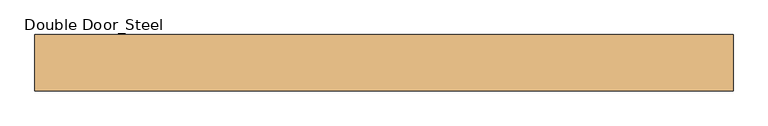
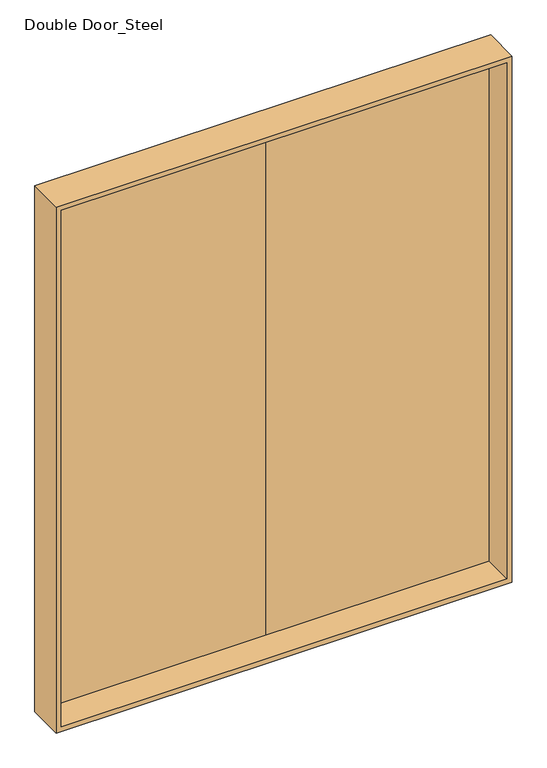
"""IFC4 building model written with IfcOpenShell, lengths in millimetres: door geometry, Double Door_Steel : H_DR_AR_B12_Double Door_Steel_W3100xH3780_FSD4."""

import ifcopenshell
import ifcopenshell.guid

model = None  # the IFC model being written
_history = None  # IfcOwnerHistory: only IFC2X3 demands one
_inside = {}  # id of a spatial element -> (the spatial element, [elements in it])
_under = {}  # id of a project, library or spatial element -> (it, [spatial elements below it])
_declared = {}  # id of a project -> (the project, [libraries it declares])
_typed = {}  # id of a type object -> (the type object, [elements of that type])
_made_of = {}  # id of a material, layer set ... -> (it, [elements and type objects made of it])


def new_model(schema):
    """Start an empty IFC model of exactly this schema.

    Asked for "IFC4X3", IfcOpenShell would pick the latest addendum, in which some entities
    have other attributes; the version numbers below select the first issue.
    IFC2X3 requires an IfcOwnerHistory on every rooted entity: one is made here for all.
    """
    global model, _history
    if schema == "IFC4X3":
        model = ifcopenshell.file(schema_version=(4, 3, 0, 0))
    else:
        model = ifcopenshell.file(schema=schema)
    _inside.clear()
    _under.clear()
    _declared.clear()
    _typed.clear()
    _made_of.clear()
    _history = None
    if model.schema == "IFC2X3":
        org = make("IfcOrganization", Name="unknown")
        user = make(
            "IfcPersonAndOrganization",
            ThePerson=make("IfcPerson", FamilyName="unknown"),
            TheOrganization=org,
        )
        app = make(
            "IfcApplication",
            ApplicationDeveloper=org,
            Version="unknown",
            ApplicationFullName="unknown",
            ApplicationIdentifier="unknown",
        )
        _history = make(
            "IfcOwnerHistory",
            OwningUser=user,
            OwningApplication=app,
            ChangeAction="ADDED",
            CreationDate=0,
        )
    return model


def make(cls, **values):
    """One entity of the class cls with the attributes given. An attribute that is None is left unset."""
    return model.create_entity(
        cls, **{name: value for name, value in values.items() if value is not None}
    )


def rooted(cls, **values):
    """An entity with a GlobalId (a new one), such as an element, a storey or a relation."""
    return make(cls, GlobalId=ifcopenshell.guid.new(), OwnerHistory=_history, **values)


def si_unit(unit_type, name, prefix=None):
    """IfcSIUnit, for example si_unit("LENGTHUNIT", "METRE", prefix="MILLI")."""
    return make("IfcSIUnit", UnitType=unit_type, Prefix=prefix, Name=name)


def assignment(units):
    """IfcUnitAssignment: the units of a project."""
    return None if units is None else make("IfcUnitAssignment", Units=units)


def point(xyz):
    """IfcCartesianPoint."""
    return None if xyz is None else make("IfcCartesianPoint", Coordinates=xyz)


def direction(xyz):
    """IfcDirection."""
    return None if xyz is None else make("IfcDirection", DirectionRatios=xyz)


def frame(location, z_axis=None, x_axis=None):
    """IfcAxis2Placement3D, a coordinate frame: its origin and axes. An axis left out is left unset."""
    return make(
        "IfcAxis2Placement3D",
        Location=point(location),
        Axis=direction(z_axis),
        RefDirection=direction(x_axis),
    )


def origin():
    """The frame at (0, 0, 0) with its axes left unset."""
    return frame((0.0, 0.0, 0.0))


def place(relative_to, where):
    """IfcLocalPlacement: puts the frame where relative to a parent placement (None: the world)."""
    return make(
        "IfcLocalPlacement", PlacementRelTo=relative_to, RelativePlacement=where
    )


def context(
    kind, dimensions, precision=None, world=None, true_north=None, identifier=None
):
    """IfcGeometricRepresentationContext, for example the 3D "Model" context."""
    return make(
        "IfcGeometricRepresentationContext",
        ContextIdentifier=identifier,
        ContextType=kind,
        CoordinateSpaceDimension=dimensions,
        Precision=precision,
        WorldCoordinateSystem=world,
        TrueNorth=true_north,
    )


def project(units=None, contexts=None):
    """IfcProject with its units and contexts."""
    return rooted(
        "IfcProject",
        Name="project",
        RepresentationContexts=contexts,
        UnitsInContext=assignment(units),
    )


def spatial(cls, under=None, at=None, **own):
    """A site, building, storey or space (cls), placed at a placement, below another one or the project."""
    s = rooted(cls, ObjectPlacement=at, **own)
    if under is not None:
        _under.setdefault(under.id(), (under, []))[1].append(s)
    return s


def polyline(points):
    """IfcPolyline through the points."""
    return make("IfcPolyline", Points=[point(p) for p in points])


def outline(outer, holes=None, kind="AREA"):
    """IfcArbitraryClosedProfileDef: a profile drawn as a closed curve; with holes, ...WithVoids."""
    if holes is None:
        return make("IfcArbitraryClosedProfileDef", ProfileType=kind, OuterCurve=outer)
    return make(
        "IfcArbitraryProfileDefWithVoids",
        ProfileType=kind,
        OuterCurve=outer,
        InnerCurves=holes,
    )


def extrude(swept, where, along, depth):
    """IfcExtrudedAreaSolid: the profile swept, set in the frame where, extruded along a direction by depth."""
    return make(
        "IfcExtrudedAreaSolid",
        SweptArea=swept,
        Position=where,
        ExtrudedDirection=direction(along),
        Depth=depth,
    )


def faces_of(points, faces, orient=None, outer=None):
    """IfcFace entities. A face is a list of loops; a loop is a list of indices into points, from 0.

    orient and outer hold one flag for each loop. By default every Orientation is true, the
    first loop of a face is its IfcFaceOuterBound and the others are IfcFaceBound.
    """
    made = []
    for i, loops in enumerate(faces):
        bounds = []
        for j, loop in enumerate(loops):
            is_outer = j == 0 if outer is None else outer[i][j]
            bounds.append(
                make(
                    "IfcFaceOuterBound" if is_outer else "IfcFaceBound",
                    Bound=make("IfcPolyLoop", Polygon=[points[k] for k in loop]),
                    Orientation=True if orient is None else orient[i][j],
                )
            )
        made.append(make("IfcFace", Bounds=bounds))
    return made


def faceted_brep(points, faces, orient=None, outer=None, voids=None):
    """IfcFacetedBrep: a solid bounded by flat faces; with voids (closed shells), ...WithVoids."""
    shared = [point(p) for p in points]
    hull = make("IfcClosedShell", CfsFaces=faces_of(shared, faces, orient, outer))
    if voids is None:
        return make("IfcFacetedBrep", Outer=hull)
    return make(
        "IfcFacetedBrepWithVoids",
        Outer=hull,
        Voids=[
            make(cls, CfsFaces=faces_of(shared, fs, o, b)) for cls, fs, o, b in voids
        ],
    )


def shape(context_of_items, identifier, shape_type, items):
    """IfcShapeRepresentation: the items that make up one representation, for example the "Body"."""
    return make(
        "IfcShapeRepresentation",
        ContextOfItems=context_of_items,
        RepresentationIdentifier=identifier,
        RepresentationType=shape_type,
        Items=items,
    )


def source(mapping_origin, context_of_items, identifier, shape_type, items):
    """IfcRepresentationMap: a shape defined once, which mapped items show again and again."""
    return make(
        "IfcRepresentationMap",
        MappingOrigin=mapping_origin,
        MappedRepresentation=shape(context_of_items, identifier, shape_type, items),
    )


def transform(
    local_origin,
    x_axis=None,
    y_axis=None,
    z_axis=None,
    scale=None,
    scale2=None,
    scale3=None,
    uniform=True,
):
    """IfcCartesianTransformationOperator3D, or its non-uniform kind. x_axis, y_axis, z_axis: its Axis1, 2, 3."""
    if uniform:
        return make(
            "IfcCartesianTransformationOperator3D",
            Axis1=direction(x_axis),
            Axis2=direction(y_axis),
            LocalOrigin=point(local_origin),
            Scale=scale,
            Axis3=direction(z_axis),
        )
    return make(
        "IfcCartesianTransformationOperator3DnonUniform",
        Axis1=direction(x_axis),
        Axis2=direction(y_axis),
        LocalOrigin=point(local_origin),
        Scale=scale,
        Axis3=direction(z_axis),
        Scale2=scale2,
        Scale3=scale3,
    )


def mapped(mapping_source, mapping_target):
    """IfcMappedItem: shows the shape of a source again, moved by a transform."""
    return make(
        "IfcMappedItem", MappingSource=mapping_source, MappingTarget=mapping_target
    )


def made_of(thing, what):
    """Note that an element or type object is made of a material, layer set ...; save() writes the relation."""
    if what is not None:
        _made_of.setdefault(what.id(), (what, []))[1].append(thing)
    return thing


def element(
    cls,
    number,
    at=None,
    inside=None,
    cuts=None,
    type_object=None,
    material=None,
    context=None,
    identifier="Body",
    shape_type=None,
    held_by="IfcProductDefinitionShape",
    body=None,
    shapes=None,
    **own,
):
    """One element of the class cls, such as IfcWall. Its Tag is "e" and its number.

    at: its placement. inside: the storey or other place that contains it. cuts: it is an
    opening in that element (IfcRelVoidsElement). A single representation is given by context,
    identifier, shape_type and body (its items); several are given by shapes. held_by: the class
    of the entity that holds the representations. save() writes the other relations.
    """
    e = rooted(cls, Tag="e%d" % number, ObjectPlacement=at, **own)
    if body is not None:
        shapes = [shape(context, identifier, shape_type, body)]
    if shapes is not None:
        e.Representation = make(held_by, Representations=shapes)
    if inside is not None:
        _inside.setdefault(inside.id(), (inside, []))[1].append(e)
    if cuts is not None:
        rooted(
            "IfcRelVoidsElement", RelatingBuildingElement=cuts, RelatedOpeningElement=e
        )
    if type_object is not None:
        _typed.setdefault(type_object.id(), (type_object, []))[1].append(e)
    return made_of(e, material)


def aggregate(whole, parts):
    """IfcRelAggregates: a whole, such as a stair, and the parts it consists of."""
    return rooted("IfcRelAggregates", RelatingObject=whole, RelatedObjects=parts)


def save(model, path):
    """Write the relations noted so far, then the file.

    IfcRelAggregates (storeys below a building ...), IfcRelContainedInSpatialStructure (elements
    in a storey), IfcRelDefinesByType, IfcRelAssociatesMaterial and IfcRelDeclares: one each for
    every whole, place, type object, material and project.
    """
    for whole, parts in _under.values():
        aggregate(whole, parts)
    for where, things in _inside.values():
        rooted(
            "IfcRelContainedInSpatialStructure",
            RelatedElements=things,
            RelatingStructure=where,
        )
    for kind, things in _typed.values():
        rooted("IfcRelDefinesByType", RelatedObjects=things, RelatingType=kind)
    for what, things in _made_of.values():
        rooted("IfcRelAssociatesMaterial", RelatedObjects=things, RelatingMaterial=what)
    for by, libraries in _declared.values():
        rooted("IfcRelDeclares", RelatingContext=by, RelatedDefinitions=libraries)
    model.write(path)


def double_door_steel_fbc497f4(model_context):
    return source(origin(), model_context, "Body", "SolidModel", [
        extrude(outline(polyline([(1530.0, 85.0), (0.0, 85.0), (0.0, 125.0), (1530.0, 125.0), (1530.0, 85.0)])), frame((0.0, 0.0, 20.0), z_axis=(0.0, 0.0, 1.0), x_axis=(1.0, 0.0, 0.0)), (0.0, 0.0, 1.0), 3740.0),
        extrude(outline(polyline([(0.0, 85.0), (-1530.0, 85.0), (-1530.0, 125.0), (0.0, 125.0), (0.0, 85.0)])), frame((0.0, 0.0, 20.0), z_axis=(0.0, 0.0, 1.0), x_axis=(1.0, 0.0, 0.0)), (0.0, 0.0, 1.0), 3740.0),
        faceted_brep([(1550.0, -125.0, 3780.0), (1550.0, 125.0, 3780.0), (-1550.0, 125.0, 3780.0), (-1550.0, -125.0, 3780.0), (1515.0, 85.0, 3745.0), (1515.0, -125.0, 3745.0), (-1515.0, -125.0, 3745.0), (-1515.0, 85.0, 3745.0), (1530.0, 125.0, 3760.0), (1530.0, 85.0, 3760.0), (-1530.0, 85.0, 3760.0), (-1530.0, 125.0, 3760.0), (-1550.0, 125.0, 0.0), (-1550.0, -125.0, 0.0), (-1515.0, -125.0, 35.0), (-1515.0, 85.0, 35.0), (-1530.0, 85.0, 20.0), (-1530.0, 125.0, 20.0), (1550.0, 125.0, 0.0), (1530.0, 125.0, 20.0), (1550.0, -125.0, 0.0), (1515.0, -125.0, 35.0), (1515.0, 85.0, 35.0), (1530.0, 85.0, 20.0)], [[[0, 1, 2, 3]], [[4, 5, 6, 7]], [[8, 9, 10, 11]], [[3, 2, 12, 13]], [[7, 6, 14, 15]], [[11, 10, 16, 17]], [[18, 12, 2, 1], [8, 11, 17, 19]], [[13, 12, 18, 20]], [[0, 3, 13, 20], [21, 14, 6, 5]], [[15, 14, 21, 22]], [[23, 16, 10, 9], [4, 7, 15, 22]], [[17, 16, 23, 19]], [[20, 18, 1, 0]], [[22, 21, 5, 4]], [[19, 23, 9, 8]]]),
    ])


if __name__ == "__main__":
    model = new_model("IFC4")
    model_context = context("Model", 3, world=origin())
    ifc_project = project(units=[si_unit("LENGTHUNIT", "METRE", prefix="MILLI")], contexts=[model_context])
    site = spatial("IfcSite", under=ifc_project)
    building = spatial("IfcBuilding", under=site)
    placement = place(None, origin())
    double_door_steel_shape = double_door_steel_fbc497f4(model_context)
    element("IfcDoor", 1, ObjectType="Double Door_Steel : H_DR_AR_B12_Double Door_Steel_W3100xH3780_FSD4", at=placement, inside=building, context=model_context, shape_type="MappedRepresentation", body=[
        mapped(double_door_steel_shape, transform((0.0, 0.0, 0.0), x_axis=(1.0, 0.0, 0.0), y_axis=(0.0, 1.0, 0.0), z_axis=(0.0, 0.0, 1.0))),
    ])
    save(model, "model.ifc")

# Revit data of these elements
# Type "Double Door_Steel : H_DR_AR_B12_Double Door_Steel_W3100xH3780_FSD4"
#   Type Mark = "442"
#   프레임 = ""
#   철물 = ""
#   유리/마감 = ""
#   위치/개소 = ""
#   부호 = "1/SD"
#   문번호 = "4"
#   문기호 = "FSD"
#   Analytic Construction = "<None>"
#   Height = 3780 mm
#   Width = 3100 mm
#   Define Thermal Properties by = 1
#   문 틀 = none
#   문 = none
#   Function = (empty or 0)
#   Assembly Code = ""
#   Wall Closure = (empty or 0)
